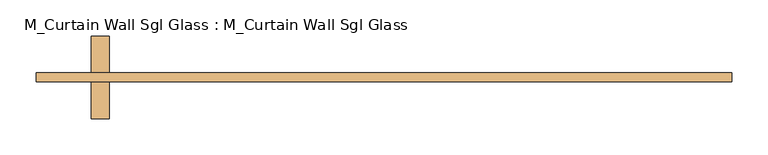
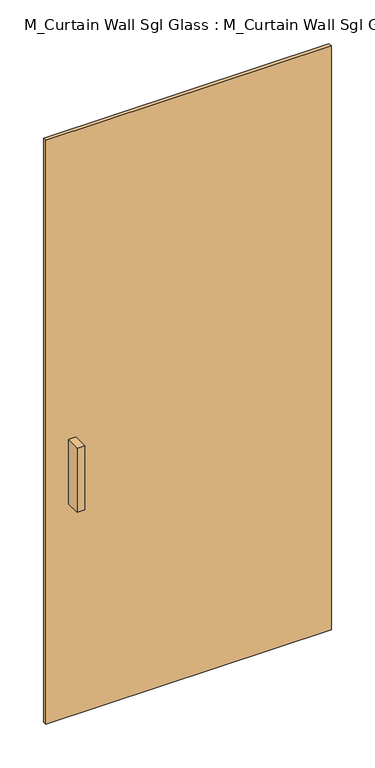
"""IFC4 building model written with IfcOpenShell, lengths in millimetres: door geometry, M_Curtain Wall Sgl Glass : M_Curtain Wall Sgl Glass."""

from ifc_helpers import new_model, si_unit, frame, origin, origin_with_axes, place, context, project, spatial, polyline, outline, extrude, source, transform, mapped, element, save


def m_curtain_wall_sgl_glass_m_curtain_wall_sgl_glass_bf48fc07(model_context):
    return source(origin(), model_context, "Body", "SweptSolid", [
        extrude(outline(polyline([(-380.9, 12.5), (-380.9, -38.3), (-406.3, -38.3), (-406.3, 12.5), (-380.9, 12.5)])), frame((0.0, 0.0, 762.0), z_axis=(0.0, 0.0, 1.0), x_axis=(1.0, 0.0, 0.0)), (0.0, 0.0, 1.0), 228.6),
        extrude(outline(polyline([(-406.3, -101.8), (-406.3, -51.0), (-380.9, -51.0), (-380.9, -101.8), (-406.3, -101.8)])), frame((0.0, 0.0, 762.0), z_axis=(0.0, 0.0, 1.0), x_axis=(1.0, 0.0, 0.0)), (0.0, 0.0, 1.0), 228.6),
        extrude(outline(polyline([(482.5, -51.0), (-482.5, -51.0), (-482.5, -38.3), (482.5, -38.3), (482.5, -51.0)])), origin_with_axes(), (0.0, 0.0, 1.0), 2085.0),
    ])


if __name__ == "__main__":
    model = new_model("IFC4")
    model_context = context("Model", 3, world=origin())
    ifc_project = project(units=[si_unit("LENGTHUNIT", "METRE", prefix="MILLI")], contexts=[model_context])
    site = spatial("IfcSite", under=ifc_project)
    building = spatial("IfcBuilding", under=site)
    placement = place(None, origin())
    m_curtain_wall_sgl_glass_m_curtain_wall_sgl_glass_shape = m_curtain_wall_sgl_glass_m_curtain_wall_sgl_glass_bf48fc07(model_context)
    element("IfcDoor", 1, ObjectType="M_Curtain Wall Sgl Glass : M_Curtain Wall Sgl Glass", at=placement, inside=building, context=model_context, shape_type="MappedRepresentation", body=[
        mapped(m_curtain_wall_sgl_glass_m_curtain_wall_sgl_glass_shape, transform((0.0, 0.0, 0.0), x_axis=(1.0, 0.0, 0.0), y_axis=(0.0, 1.0, 0.0), z_axis=(0.0, 0.0, 1.0))),
    ])
    save(model, "model.ifc")

# Revit data of these elements
# Type "M_Curtain Wall Sgl Glass : M_Curtain Wall Sgl Glass"
#   Type Mark = "40"
#   COBie.Type.CreatedBy = "design@eagle.com"
#   COBie.Type.CreatedOn = "2016-09-13T05:47:35"
#   COBie.Type.Name = "Doors_M_Curtain Wall Sgl Glass_M_Curtain Wall Sgl Glass"
#   COBie.Type.Category = "23-30 10 00 : Doors"
#   COBie.Type.Description = ""
#   COBie.Type.Manufacturer = ""
#   COBie.Type.ModelNumber = ""
#   Construction Type Id = "SGL"
#   Analytic Construction = "Large single-glazed windows"
#   COBie.Type.ReplacementCost = 0
#   Visual Light Transmittance = 0.9
#   Solar Heat Gain Coefficient = 0.86
#   Offset = 51 mm
#   Heat Transfer Coefficient (U) = 5.5617 W/(m²·K)
#   COBie.Type = yes
#   Function = 1
#   Glazing Material = Glass
# Element 1 (IfcDoor, "M_Curtain Wall Sgl Glass : M_Curtain Wall Sgl Glass")
#   Materials on its faces: "Aluminum", "Glass"
# Materials
#   "Glass": class "Glass", colour RGB 0 128 192, transparency 0.75, Description = "Soda Lime Glass", Cost = 0
#   "Aluminum": class "Metal", colour RGB 247 247 247, transparency 0, Description = "Aluminum 6061", Cost = 0
